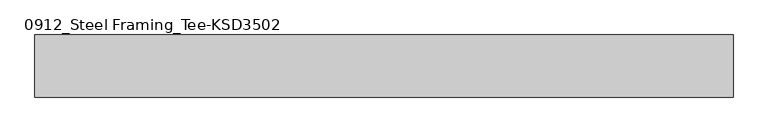
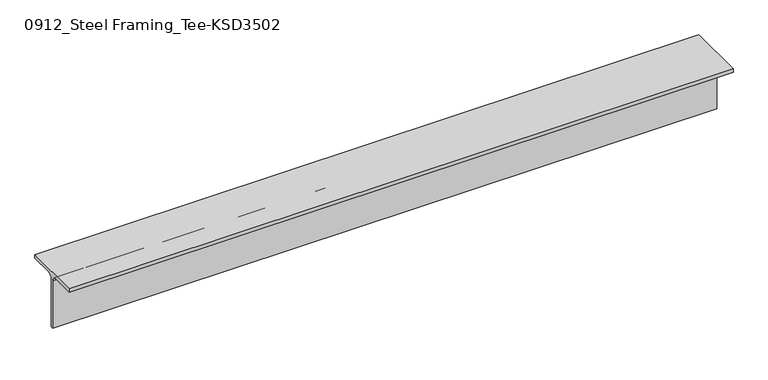
"""IFC4 building model written with IfcOpenShell, lengths in millimetres: member geometry, 0912_Steel Framing_Tee-KSD3502 : H_SB_ASB_CT-150x150x6.5x9."""

from ifc_helpers import new_model, si_unit, point, frame, frame_2d, origin, place, context, project, spatial, polyline, circle_curve, trimmed, segment, composite_curve, outline, extrude, source, transform, mapped, element, save


def member_0912_steel_framing_tee_ksd3502_28f52639(model_context):
    return source(origin(), model_context, "Body", "SweptSolid", [
        extrude(outline(composite_curve([segment(polyline([(-75.0, 75.0), (75.0, 75.0), (75.0, 66.0), (16.25, 66.0)]), True, "CONTINUOUS"), segment(trimmed(circle_curve(frame_2d((16.25, 53.0)), 13.0), [point((16.25, 66.0))], [point((3.25, 53.0))], True, "CARTESIAN"), True, "CONTINUOUS"), segment(polyline([(3.25, 53.0), (3.25, -75.0), (-3.25, -75.0), (-3.25, 53.0)]), True, "CONTINUOUS"), segment(trimmed(circle_curve(frame_2d((-16.25, 53.0)), 13.0), [point((-3.25, 53.0))], [point((-16.25, 66.0))], True, "CARTESIAN"), True, "CONTINUOUS"), segment(polyline([(-16.25, 66.0), (-75.0, 66.0), (-75.0, 75.0)]), True, "CONTINUOUS")], self_intersect=False)), frame((-842.3, 0.0, 0.0), z_axis=(1.0, 0.0, 0.0), x_axis=(0.0, 1.0, 0.0)), (0.0, 0.0, 1.0), 1684.6),
    ])


if __name__ == "__main__":
    model = new_model("IFC4")
    model_context = context("Model", 3, world=origin())
    ifc_project = project(units=[si_unit("LENGTHUNIT", "METRE", prefix="MILLI")], contexts=[model_context])
    site = spatial("IfcSite", under=ifc_project)
    building = spatial("IfcBuilding", under=site)
    placement = place(None, origin())
    member_0912_steel_framing_tee_ksd3502_shape = member_0912_steel_framing_tee_ksd3502_28f52639(model_context)
    element("IfcMember", 1, ObjectType="0912_Steel Framing_Tee-KSD3502 : H_SB_ASB_CT-150x150x6.5x9", at=placement, inside=building, context=model_context, shape_type="MappedRepresentation", body=[
        mapped(member_0912_steel_framing_tee_ksd3502_shape, transform((0.0, 0.0, 0.0), x_axis=(1.0, 0.0, 0.0), y_axis=(0.0, 1.0, 0.0), z_axis=(0.0, 0.0, 1.0))),
    ])
    save(model, "model.ifc")

# Revit data of these elements
# Type "0912_Steel Framing_Tee-KSD3502 : H_SB_ASB_CT-150x150x6.5x9"
#   H_WM Code_1 = "S01AA003-00001 | Main Steel Structure Fabrication Work | Shelter/Building | Light Steel - Standard (30KG/M>Weight) | Material: (   )"
#   H_WM Code_2 = "S03AA029-00001 | Main Steel Structure Erection Work | Shelter/Building | Light Steel (30KG/M>Weight) | Material: (   )"
#   H_WM Code_3 = "S01AA010-00001 | Main Steel Structure Fabrication Work | Shelter/Building | Steel Painting/Coating | for Non-Fireproofed Steel Surface, Surface Preparation, Primer, Second & Final Coat | Material: (   )"
#   H_Q'ty Cal Type Tag = "SB-Q2"
#   Width = 15.0 cm
#   Web Thickness = 0.65 cm
#   Web Fillet = 1.3 cm
#   Section Area = 23.39 cm²
#   Perimeter = 0.60 m²/m
#   Nominal Weight = 18.40 kgf/m
#   Height = 15.0 cm
#   Flange Thickness = 0.9 cm
#   Centroid Vertical = 7.5 cm
#   Centroid Horizontal = 7.5 cm
#   Length [instance default] = 1.5000 m
#   Structural Material [instance default] = Steel, 45-345
#   Warping Constant = (empty or 0)
#   Torsional Moment of Inertia = 0
#   Section Name Key = ""
#   Plastic Modulus weak axis = 0
#   Plastic Modulus strong axis = 0
#   Moment of Inertia weak axis = 0
#   Moment of Inertia strong axis = 0
#   Elastic Modulus weak axis = 0
#   Elastic Modulus strong axis = 0
#   Bolt Spacing = 0
#   Assembly Code = ""
# Element 1 (IfcMember, "0912_Steel Framing_Tee-KSD3502 : H_SB_ASB_CT-150x150x6.5x9")
#   Structural Material = none
# Materials
#   "Steel, 45-345": class "Metal", colour RGB 189 187 185, transparency 0, Description = "Steel 345 MPa", Cost = 0
